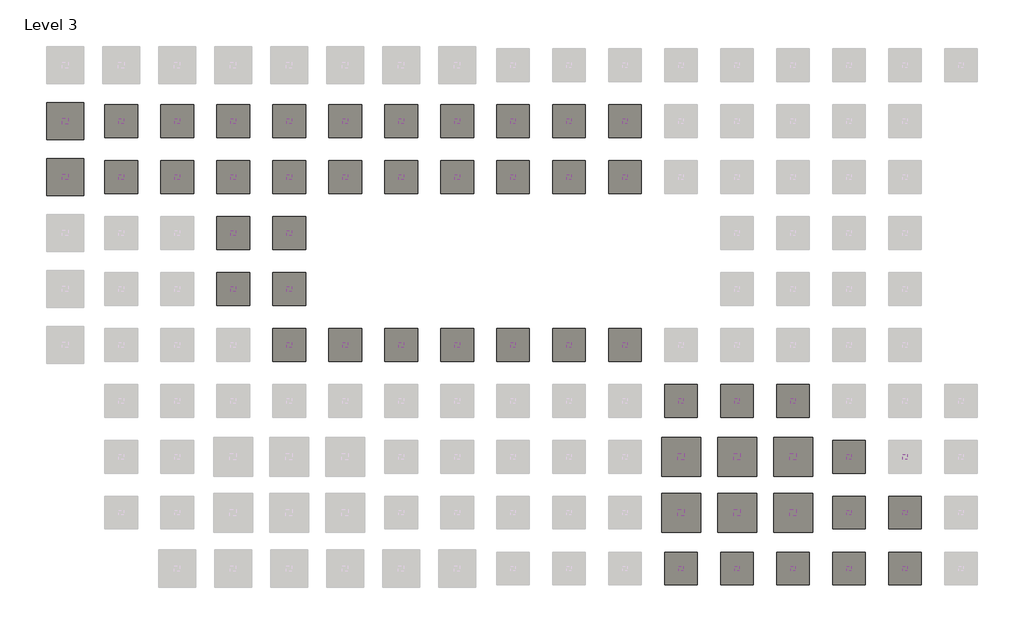
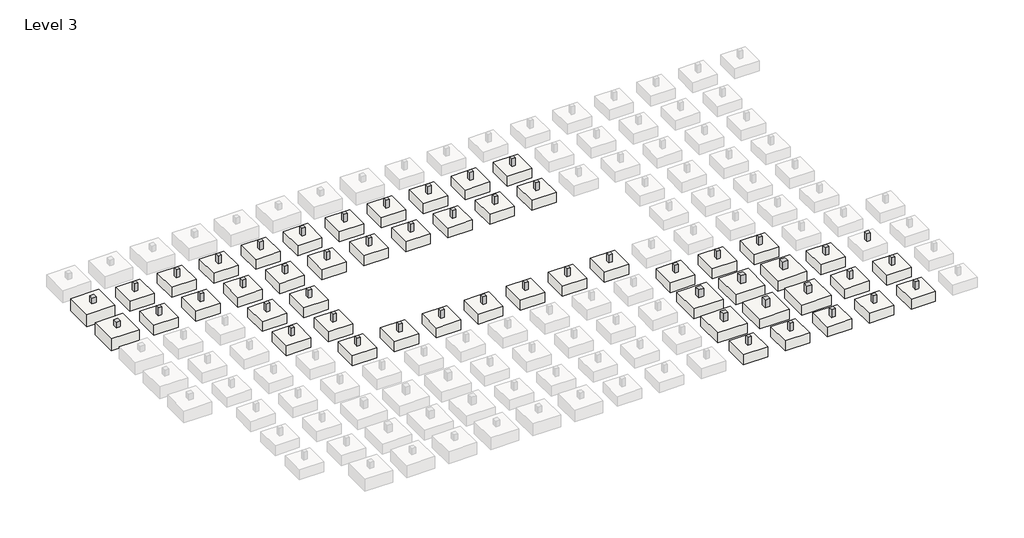
# One storey, part 2 of 3: 51 columns, 50 slabs.
"""IFC4 building model written with IfcOpenShell, lengths in millimetres."""

import ifcopenshell
import ifcopenshell.guid

model = None  # the IFC model being written
_history = None  # IfcOwnerHistory: only IFC2X3 demands one
_inside = {}  # id of a spatial element -> (the spatial element, [elements in it])
_under = {}  # id of a project, library or spatial element -> (it, [spatial elements below it])
_declared = {}  # id of a project -> (the project, [libraries it declares])
_typed = {}  # id of a type object -> (the type object, [elements of that type])
_made_of = {}  # id of a material, layer set ... -> (it, [elements and type objects made of it])


def new_model(schema):
    """Start an empty IFC model of exactly this schema.

    Asked for "IFC4X3", IfcOpenShell would pick the latest addendum, in which some entities
    have other attributes; the version numbers below select the first issue.
    IFC2X3 requires an IfcOwnerHistory on every rooted entity: one is made here for all.
    """
    global model, _history
    if schema == "IFC4X3":
        model = ifcopenshell.file(schema_version=(4, 3, 0, 0))
    else:
        model = ifcopenshell.file(schema=schema)
    _inside.clear()
    _under.clear()
    _declared.clear()
    _typed.clear()
    _made_of.clear()
    _history = None
    if model.schema == "IFC2X3":
        org = make("IfcOrganization", Name="unknown")
        user = make(
            "IfcPersonAndOrganization",
            ThePerson=make("IfcPerson", FamilyName="unknown"),
            TheOrganization=org,
        )
        app = make(
            "IfcApplication",
            ApplicationDeveloper=org,
            Version="unknown",
            ApplicationFullName="unknown",
            ApplicationIdentifier="unknown",
        )
        _history = make(
            "IfcOwnerHistory",
            OwningUser=user,
            OwningApplication=app,
            ChangeAction="ADDED",
            CreationDate=0,
        )
    return model


def make(cls, **values):
    """One entity of the class cls with the attributes given. An attribute that is None is left unset."""
    return model.create_entity(
        cls, **{name: value for name, value in values.items() if value is not None}
    )


def rooted(cls, **values):
    """An entity with a GlobalId (a new one), such as an element, a storey or a relation."""
    return make(cls, GlobalId=ifcopenshell.guid.new(), OwnerHistory=_history, **values)


def si_unit(unit_type, name, prefix=None):
    """IfcSIUnit, for example si_unit("LENGTHUNIT", "METRE", prefix="MILLI")."""
    return make("IfcSIUnit", UnitType=unit_type, Prefix=prefix, Name=name)


def assignment(units):
    """IfcUnitAssignment: the units of a project."""
    return None if units is None else make("IfcUnitAssignment", Units=units)


def point(xyz):
    """IfcCartesianPoint."""
    return None if xyz is None else make("IfcCartesianPoint", Coordinates=xyz)


def direction(xyz):
    """IfcDirection."""
    return None if xyz is None else make("IfcDirection", DirectionRatios=xyz)


def frame(location, z_axis=None, x_axis=None):
    """IfcAxis2Placement3D, a coordinate frame: its origin and axes. An axis left out is left unset."""
    return make(
        "IfcAxis2Placement3D",
        Location=point(location),
        Axis=direction(z_axis),
        RefDirection=direction(x_axis),
    )


def origin():
    """The frame at (0, 0, 0) with its axes left unset."""
    return frame((0.0, 0.0, 0.0))


def origin_with_axes():
    """The frame at (0, 0, 0) with the z axis (0, 0, 1) and the x axis (1, 0, 0) written out."""
    return frame((0.0, 0.0, 0.0), z_axis=(0.0, 0.0, 1.0), x_axis=(1.0, 0.0, 0.0))


def place(relative_to, where):
    """IfcLocalPlacement: puts the frame where relative to a parent placement (None: the world)."""
    return make(
        "IfcLocalPlacement", PlacementRelTo=relative_to, RelativePlacement=where
    )


def context(
    kind, dimensions, precision=None, world=None, true_north=None, identifier=None
):
    """IfcGeometricRepresentationContext, for example the 3D "Model" context."""
    return make(
        "IfcGeometricRepresentationContext",
        ContextIdentifier=identifier,
        ContextType=kind,
        CoordinateSpaceDimension=dimensions,
        Precision=precision,
        WorldCoordinateSystem=world,
        TrueNorth=true_north,
    )


def project(units=None, contexts=None):
    """IfcProject with its units and contexts."""
    return rooted(
        "IfcProject",
        Name="project",
        RepresentationContexts=contexts,
        UnitsInContext=assignment(units),
    )


def spatial(cls, under=None, at=None, **own):
    """A site, building, storey or space (cls), placed at a placement, below another one or the project."""
    s = rooted(cls, ObjectPlacement=at, **own)
    if under is not None:
        _under.setdefault(under.id(), (under, []))[1].append(s)
    return s


def polyline(points):
    """IfcPolyline through the points."""
    return make("IfcPolyline", Points=[point(p) for p in points])


def outline(outer, holes=None, kind="AREA"):
    """IfcArbitraryClosedProfileDef: a profile drawn as a closed curve; with holes, ...WithVoids."""
    if holes is None:
        return make("IfcArbitraryClosedProfileDef", ProfileType=kind, OuterCurve=outer)
    return make(
        "IfcArbitraryProfileDefWithVoids",
        ProfileType=kind,
        OuterCurve=outer,
        InnerCurves=holes,
    )


def extrude(swept, where, along, depth):
    """IfcExtrudedAreaSolid: the profile swept, set in the frame where, extruded along a direction by depth."""
    return make(
        "IfcExtrudedAreaSolid",
        SweptArea=swept,
        Position=where,
        ExtrudedDirection=direction(along),
        Depth=depth,
    )


def shape(context_of_items, identifier, shape_type, items):
    """IfcShapeRepresentation: the items that make up one representation, for example the "Body"."""
    return make(
        "IfcShapeRepresentation",
        ContextOfItems=context_of_items,
        RepresentationIdentifier=identifier,
        RepresentationType=shape_type,
        Items=items,
    )


def source(mapping_origin, context_of_items, identifier, shape_type, items):
    """IfcRepresentationMap: a shape defined once, which mapped items show again and again."""
    return make(
        "IfcRepresentationMap",
        MappingOrigin=mapping_origin,
        MappedRepresentation=shape(context_of_items, identifier, shape_type, items),
    )


def transform(
    local_origin,
    x_axis=None,
    y_axis=None,
    z_axis=None,
    scale=None,
    scale2=None,
    scale3=None,
    uniform=True,
):
    """IfcCartesianTransformationOperator3D, or its non-uniform kind. x_axis, y_axis, z_axis: its Axis1, 2, 3."""
    if uniform:
        return make(
            "IfcCartesianTransformationOperator3D",
            Axis1=direction(x_axis),
            Axis2=direction(y_axis),
            LocalOrigin=point(local_origin),
            Scale=scale,
            Axis3=direction(z_axis),
        )
    return make(
        "IfcCartesianTransformationOperator3DnonUniform",
        Axis1=direction(x_axis),
        Axis2=direction(y_axis),
        LocalOrigin=point(local_origin),
        Scale=scale,
        Axis3=direction(z_axis),
        Scale2=scale2,
        Scale3=scale3,
    )


def mapped(mapping_source, mapping_target):
    """IfcMappedItem: shows the shape of a source again, moved by a transform."""
    return make(
        "IfcMappedItem", MappingSource=mapping_source, MappingTarget=mapping_target
    )


def made_of(thing, what):
    """Note that an element or type object is made of a material, layer set ...; save() writes the relation."""
    if what is not None:
        _made_of.setdefault(what.id(), (what, []))[1].append(thing)
    return thing


def element(
    cls,
    number,
    at=None,
    inside=None,
    cuts=None,
    type_object=None,
    material=None,
    context=None,
    identifier="Body",
    shape_type=None,
    held_by="IfcProductDefinitionShape",
    body=None,
    shapes=None,
    **own,
):
    """One element of the class cls, such as IfcWall. Its Tag is "e" and its number.

    at: its placement. inside: the storey or other place that contains it. cuts: it is an
    opening in that element (IfcRelVoidsElement). A single representation is given by context,
    identifier, shape_type and body (its items); several are given by shapes. held_by: the class
    of the entity that holds the representations. save() writes the other relations.
    """
    e = rooted(cls, Tag="e%d" % number, ObjectPlacement=at, **own)
    if body is not None:
        shapes = [shape(context, identifier, shape_type, body)]
    if shapes is not None:
        e.Representation = make(held_by, Representations=shapes)
    if inside is not None:
        _inside.setdefault(inside.id(), (inside, []))[1].append(e)
    if cuts is not None:
        rooted(
            "IfcRelVoidsElement", RelatingBuildingElement=cuts, RelatedOpeningElement=e
        )
    if type_object is not None:
        _typed.setdefault(type_object.id(), (type_object, []))[1].append(e)
    return made_of(e, material)


def aggregate(whole, parts):
    """IfcRelAggregates: a whole, such as a stair, and the parts it consists of."""
    return rooted("IfcRelAggregates", RelatingObject=whole, RelatedObjects=parts)


def save(model, path):
    """Write the relations noted so far, then the file.

    IfcRelAggregates (storeys below a building ...), IfcRelContainedInSpatialStructure (elements
    in a storey), IfcRelDefinesByType, IfcRelAssociatesMaterial and IfcRelDeclares: one each for
    every whole, place, type object, material and project.
    """
    for whole, parts in _under.values():
        aggregate(whole, parts)
    for where, things in _inside.values():
        rooted(
            "IfcRelContainedInSpatialStructure",
            RelatedElements=things,
            RelatingStructure=where,
        )
    for kind, things in _typed.values():
        rooted("IfcRelDefinesByType", RelatedObjects=things, RelatingType=kind)
    for what, things in _made_of.values():
        rooted("IfcRelAssociatesMaterial", RelatedObjects=things, RelatingMaterial=what)
    for by, libraries in _declared.values():
        rooted("IfcRelDeclares", RelatingContext=by, RelatedDefinitions=libraries)
    model.write(path)


def cl111_concrete_rectangular_column_cl111_500x500_13a722a7(model_context):
    return source(origin(), model_context, "Body", "SweptSolid", [
        extrude(outline(polyline([(250.0, 250.0), (250.0, -250.0), (-250.0, -250.0), (-250.0, 250.0), (250.0, 250.0)])), frame((0.0, 0.0, -1200.0), z_axis=(0.0, 0.0, 1.0), x_axis=(1.0, 0.0, 0.0)), (0.0, 0.0, 1.0), 1200.0),
    ])


def cl111_concrete_rectangular_column_cl111_700x700_c1bab047(model_context):
    return source(origin(), model_context, "Body", "SweptSolid", [
        extrude(outline(polyline([(350.0, 350.0), (350.0, -350.0), (-350.0, -350.0), (-350.0, 350.0), (350.0, 350.0)])), frame((0.0, 0.0, -1200.0), z_axis=(0.0, 0.0, 1.0), x_axis=(1.0, 0.0, 0.0)), (0.0, 0.0, 1.0), 1200.0),
    ])


def ft111_footing_rectangular_ft111_3500x3500_d0491e67(model_context):
    return source(origin(), model_context, "Body", "SweptSolid", [
        extrude(outline(polyline([(1750.0, 1750.0), (1750.0, -1750.0), (-1750.0, -1750.0), (-1750.0, 1750.0), (1750.0, 1750.0)])), origin_with_axes(), (0.0, 0.0, 1.0), 1500.0),
    ])


def ft111_footing_rectangular_ft111_4200x4200_1dfe1a53(model_context):
    return source(origin(), model_context, "Body", "SweptSolid", [
        extrude(outline(polyline([(2100.0, 2100.0), (2100.0, -2100.0), (-2100.0, -2100.0), (-2100.0, 2100.0), (2100.0, 2100.0)])), origin_with_axes(), (0.0, 0.0, 1.0), 1500.0),
    ])


model = new_model("IFC4")

# Units and contexts
model_context = context("Model", 3, world=origin())
ifc_project = project(units=[si_unit("LENGTHUNIT", "METRE", prefix="MILLI")], contexts=[model_context])

# Site, building, storey
site = spatial("IfcSite", under=ifc_project)
building = spatial("IfcBuilding", under=site)
storey = spatial("IfcBuildingStorey", under=building, Name="Level 3", Elevation=-2700.0)

# Columns
placement = place(None, origin())
element("IfcColumn", 1, ObjectType="CL111_Concrete-Rectangular-Column : CL111_500x500", at=placement, inside=storey, context=model_context, shape_type="SweptSolid", body=[
    extrude(outline(polyline([(84250.0, -53750.0), (84250.0, -54250.0), (83750.0, -54250.0), (83750.0, -53750.0), (84250.0, -53750.0)])), frame((0.0, 0.0, -1200.0), z_axis=(0.0, 0.0, 1.0), x_axis=(1.0, 0.0, 0.0)), (0.0, 0.0, 1.0), 1200.0),
])
element("IfcColumn", 2, ObjectType="CL111_Concrete-Rectangular-Column : CL111_500x500", at=placement, inside=storey, context=model_context, shape_type="SweptSolid", body=[
    extrude(outline(polyline([(90250.0, -53750.0), (90250.0, -54250.0), (89750.0, -54250.0), (89750.0, -53750.0), (90250.0, -53750.0)])), frame((0.0, 0.0, -1200.0), z_axis=(0.0, 0.0, 1.0), x_axis=(1.0, 0.0, 0.0)), (0.0, 0.0, 1.0), 1200.0),
])
element("IfcColumn", 3, ObjectType="CL111_Concrete-Rectangular-Column : CL111_500x500", at=placement, inside=storey, context=model_context, shape_type="SweptSolid", body=[
    extrude(outline(polyline([(72250.0, -53750.0), (72250.0, -54250.0), (71750.0, -54250.0), (71750.0, -53750.0), (72250.0, -53750.0)])), frame((0.0, 0.0, -1200.0), z_axis=(0.0, 0.0, 1.0), x_axis=(1.0, 0.0, 0.0)), (0.0, 0.0, 1.0), 1200.0),
])
element("IfcColumn", 4, ObjectType="CL111_Concrete-Rectangular-Column : CL111_500x500", at=placement, inside=storey, context=model_context, shape_type="SweptSolid", body=[
    extrude(outline(polyline([(78250.0, -53750.0), (78250.0, -54250.0), (77750.0, -54250.0), (77750.0, -53750.0), (78250.0, -53750.0)])), frame((0.0, 0.0, -1200.0), z_axis=(0.0, 0.0, 1.0), x_axis=(1.0, 0.0, 0.0)), (0.0, 0.0, 1.0), 1200.0),
])
element("IfcColumn", 5, ObjectType="CL111_Concrete-Rectangular-Column : CL111_500x500", at=placement, inside=storey, context=model_context, shape_type="SweptSolid", body=[
    extrude(outline(polyline([(66250.0, -53750.0), (66250.0, -54250.0), (65750.0, -54250.0), (65750.0, -53750.0), (66250.0, -53750.0)])), frame((0.0, 0.0, -1200.0), z_axis=(0.0, 0.0, 1.0), x_axis=(1.0, 0.0, 0.0)), (0.0, 0.0, 1.0), 1200.0),
])
cl111_concrete_rectangular_column_cl111_500x500_shape = cl111_concrete_rectangular_column_cl111_500x500_13a722a7(model_context)
element("IfcColumn", 6, ObjectType="CL111_Concrete-Rectangular-Column : CL111_500x500", at=placement, inside=storey, context=model_context, shape_type="MappedRepresentation", body=[
    mapped(cl111_concrete_rectangular_column_cl111_500x500_shape, transform((54000.0, -30000.0, 0.0), x_axis=(1.0, 0.0, 0.0), y_axis=(0.0, 1.0, 0.0), z_axis=(0.0, 0.0, 1.0))),
])
element("IfcColumn", 7, ObjectType="CL111_Concrete-Rectangular-Column : CL111_500x500", at=placement, inside=storey, context=model_context, shape_type="MappedRepresentation", body=[
    mapped(cl111_concrete_rectangular_column_cl111_500x500_shape, transform((54000.0, -12000.0, 0.0), x_axis=(1.0, 0.0, 0.0), y_axis=(0.0, 1.0, 0.0), z_axis=(0.0, 0.0, 1.0))),
])
element("IfcColumn", 8, ObjectType="CL111_Concrete-Rectangular-Column : CL111_500x500", at=placement, inside=storey, context=model_context, shape_type="MappedRepresentation", body=[
    mapped(cl111_concrete_rectangular_column_cl111_500x500_shape, transform((54000.0, -6000.0, 0.0), x_axis=(1.0, 0.0, 0.0), y_axis=(0.0, 1.0, 0.0), z_axis=(0.0, 0.0, 1.0))),
])
element("IfcColumn", 9, ObjectType="CL111_Concrete-Rectangular-Column : CL111_500x500", at=placement, inside=storey, context=model_context, shape_type="MappedRepresentation", body=[
    mapped(cl111_concrete_rectangular_column_cl111_500x500_shape, transform((84000.0, -48000.0, 0.0), x_axis=(1.0, 0.0, 0.0), y_axis=(0.0, 1.0, 0.0), z_axis=(0.0, 0.0, 1.0))),
])
element("IfcColumn", 10, ObjectType="CL111_Concrete-Rectangular-Column : CL111_500x500", at=placement, inside=storey, context=model_context, shape_type="MappedRepresentation", body=[
    mapped(cl111_concrete_rectangular_column_cl111_500x500_shape, transform((84000.0, -42000.0, 0.0), x_axis=(1.0, 0.0, 0.0), y_axis=(0.0, 1.0, 0.0), z_axis=(0.0, 0.0, 1.0))),
])
element("IfcColumn", 11, ObjectType="CL111_Concrete-Rectangular-Column : CL111_500x500", at=placement, inside=storey, context=model_context, shape_type="MappedRepresentation", body=[
    mapped(cl111_concrete_rectangular_column_cl111_500x500_shape, transform((18000.0, -24000.0, 0.0), x_axis=(1.0, 0.0, 0.0), y_axis=(0.0, 1.0, 0.0), z_axis=(0.0, 0.0, 1.0))),
])
element("IfcColumn", 12, ObjectType="CL111_Concrete-Rectangular-Column : CL111_500x500", at=placement, inside=storey, context=model_context, shape_type="MappedRepresentation", body=[
    mapped(cl111_concrete_rectangular_column_cl111_500x500_shape, transform((24000.0, -24000.0, 0.0), x_axis=(1.0, 0.0, 0.0), y_axis=(0.0, 1.0, 0.0), z_axis=(0.0, 0.0, 1.0))),
])
element("IfcColumn", 13, ObjectType="CL111_Concrete-Rectangular-Column : CL111_500x500", at=placement, inside=storey, context=model_context, shape_type="MappedRepresentation", body=[
    mapped(cl111_concrete_rectangular_column_cl111_500x500_shape, transform((24000.0, -18000.0, 0.0), x_axis=(1.0, 0.0, 0.0), y_axis=(0.0, 1.0, 0.0), z_axis=(0.0, 0.0, 1.0))),
])
element("IfcColumn", 14, ObjectType="CL111_Concrete-Rectangular-Column : CL111_500x500", at=placement, inside=storey, context=model_context, shape_type="MappedRepresentation", body=[
    mapped(cl111_concrete_rectangular_column_cl111_500x500_shape, transform((18000.0, -18000.0, 0.0), x_axis=(1.0, 0.0, 0.0), y_axis=(0.0, 1.0, 0.0), z_axis=(0.0, 0.0, 1.0))),
])
element("IfcColumn", 15, ObjectType="CL111_Concrete-Rectangular-Column : CL111_500x500", at=placement, inside=storey, context=model_context, shape_type="MappedRepresentation", body=[
    mapped(cl111_concrete_rectangular_column_cl111_500x500_shape, transform((36000.0, -30000.0, 0.0), x_axis=(1.0, 0.0, 0.0), y_axis=(0.0, 1.0, 0.0), z_axis=(0.0, 0.0, 1.0))),
])
element("IfcColumn", 16, ObjectType="CL111_Concrete-Rectangular-Column : CL111_500x500", at=placement, inside=storey, context=model_context, shape_type="MappedRepresentation", body=[
    mapped(cl111_concrete_rectangular_column_cl111_500x500_shape, transform((30000.0, -30000.0, 0.0), x_axis=(1.0, 0.0, 0.0), y_axis=(0.0, 1.0, 0.0), z_axis=(0.0, 0.0, 1.0))),
])
element("IfcColumn", 17, ObjectType="CL111_Concrete-Rectangular-Column : CL111_500x500", at=placement, inside=storey, context=model_context, shape_type="MappedRepresentation", body=[
    mapped(cl111_concrete_rectangular_column_cl111_500x500_shape, transform((24000.0, -30000.0, 0.0), x_axis=(1.0, 0.0, 0.0), y_axis=(0.0, 1.0, 0.0), z_axis=(0.0, 0.0, 1.0))),
])
element("IfcColumn", 18, ObjectType="CL111_Concrete-Rectangular-Column : CL111_500x500", at=placement, inside=storey, context=model_context, shape_type="MappedRepresentation", body=[
    mapped(cl111_concrete_rectangular_column_cl111_500x500_shape, transform((48000.0, -30000.0, 0.0), x_axis=(1.0, 0.0, 0.0), y_axis=(0.0, 1.0, 0.0), z_axis=(0.0, 0.0, 1.0))),
])
element("IfcColumn", 19, ObjectType="CL111_Concrete-Rectangular-Column : CL111_500x500", at=placement, inside=storey, context=model_context, shape_type="MappedRepresentation", body=[
    mapped(cl111_concrete_rectangular_column_cl111_500x500_shape, transform((42000.0, -30000.0, 0.0), x_axis=(1.0, 0.0, 0.0), y_axis=(0.0, 1.0, 0.0), z_axis=(0.0, 0.0, 1.0))),
])
element("IfcColumn", 20, ObjectType="CL111_Concrete-Rectangular-Column : CL111_500x500", at=placement, inside=storey, context=model_context, shape_type="MappedRepresentation", body=[
    mapped(cl111_concrete_rectangular_column_cl111_500x500_shape, transform((30000.0, -12000.0, 0.0), x_axis=(1.0, 0.0, 0.0), y_axis=(0.0, 1.0, 0.0), z_axis=(0.0, 0.0, 1.0))),
])
element("IfcColumn", 21, ObjectType="CL111_Concrete-Rectangular-Column : CL111_500x500", at=placement, inside=storey, context=model_context, shape_type="MappedRepresentation", body=[
    mapped(cl111_concrete_rectangular_column_cl111_500x500_shape, transform((36000.0, -12000.0, 0.0), x_axis=(1.0, 0.0, 0.0), y_axis=(0.0, 1.0, 0.0), z_axis=(0.0, 0.0, 1.0))),
])
element("IfcColumn", 22, ObjectType="CL111_Concrete-Rectangular-Column : CL111_500x500", at=placement, inside=storey, context=model_context, shape_type="MappedRepresentation", body=[
    mapped(cl111_concrete_rectangular_column_cl111_500x500_shape, transform((18000.0, -12000.0, 0.0), x_axis=(1.0, 0.0, 0.0), y_axis=(0.0, 1.0, 0.0), z_axis=(0.0, 0.0, 1.0))),
])
element("IfcColumn", 23, ObjectType="CL111_Concrete-Rectangular-Column : CL111_500x500", at=placement, inside=storey, context=model_context, shape_type="MappedRepresentation", body=[
    mapped(cl111_concrete_rectangular_column_cl111_500x500_shape, transform((24000.0, -12000.0, 0.0), x_axis=(1.0, 0.0, 0.0), y_axis=(0.0, 1.0, 0.0), z_axis=(0.0, 0.0, 1.0))),
])
element("IfcColumn", 24, ObjectType="CL111_Concrete-Rectangular-Column : CL111_500x500", at=placement, inside=storey, context=model_context, shape_type="MappedRepresentation", body=[
    mapped(cl111_concrete_rectangular_column_cl111_500x500_shape, transform((6000.0, -12000.0, 0.0), x_axis=(1.0, 0.0, 0.0), y_axis=(0.0, 1.0, 0.0), z_axis=(0.0, 0.0, 1.0))),
])
element("IfcColumn", 25, ObjectType="CL111_Concrete-Rectangular-Column : CL111_500x500", at=placement, inside=storey, context=model_context, shape_type="MappedRepresentation", body=[
    mapped(cl111_concrete_rectangular_column_cl111_500x500_shape, transform((12000.0, -12000.0, 0.0), x_axis=(1.0, 0.0, 0.0), y_axis=(0.0, 1.0, 0.0), z_axis=(0.0, 0.0, 1.0))),
])
element("IfcColumn", 26, ObjectType="CL111_Concrete-Rectangular-Column : CL111_500x500", at=placement, inside=storey, context=model_context, shape_type="MappedRepresentation", body=[
    mapped(cl111_concrete_rectangular_column_cl111_500x500_shape, transform((42000.0, -12000.0, 0.0), x_axis=(1.0, 0.0, 0.0), y_axis=(0.0, 1.0, 0.0), z_axis=(0.0, 0.0, 1.0))),
])
element("IfcColumn", 27, ObjectType="CL111_Concrete-Rectangular-Column : CL111_500x500", at=placement, inside=storey, context=model_context, shape_type="MappedRepresentation", body=[
    mapped(cl111_concrete_rectangular_column_cl111_500x500_shape, transform((48000.0, -12000.0, 0.0), x_axis=(1.0, 0.0, 0.0), y_axis=(0.0, 1.0, 0.0), z_axis=(0.0, 0.0, 1.0))),
])
element("IfcColumn", 28, ObjectType="CL111_Concrete-Rectangular-Column : CL111_500x500", at=placement, inside=storey, context=model_context, shape_type="MappedRepresentation", body=[
    mapped(cl111_concrete_rectangular_column_cl111_500x500_shape, transform((36000.0, -6000.0, 0.0), x_axis=(1.0, 0.0, 0.0), y_axis=(0.0, 1.0, 0.0), z_axis=(0.0, 0.0, 1.0))),
])
element("IfcColumn", 29, ObjectType="CL111_Concrete-Rectangular-Column : CL111_500x500", at=placement, inside=storey, context=model_context, shape_type="MappedRepresentation", body=[
    mapped(cl111_concrete_rectangular_column_cl111_500x500_shape, transform((30000.0, -6000.0, 0.0), x_axis=(1.0, 0.0, 0.0), y_axis=(0.0, 1.0, 0.0), z_axis=(0.0, 0.0, 1.0))),
])
element("IfcColumn", 30, ObjectType="CL111_Concrete-Rectangular-Column : CL111_500x500", at=placement, inside=storey, context=model_context, shape_type="MappedRepresentation", body=[
    mapped(cl111_concrete_rectangular_column_cl111_500x500_shape, transform((24000.0, -6000.0, 0.0), x_axis=(1.0, 0.0, 0.0), y_axis=(0.0, 1.0, 0.0), z_axis=(0.0, 0.0, 1.0))),
])
element("IfcColumn", 31, ObjectType="CL111_Concrete-Rectangular-Column : CL111_500x500", at=placement, inside=storey, context=model_context, shape_type="MappedRepresentation", body=[
    mapped(cl111_concrete_rectangular_column_cl111_500x500_shape, transform((18000.0, -6000.0, 0.0), x_axis=(1.0, 0.0, 0.0), y_axis=(0.0, 1.0, 0.0), z_axis=(0.0, 0.0, 1.0))),
])
element("IfcColumn", 32, ObjectType="CL111_Concrete-Rectangular-Column : CL111_500x500", at=placement, inside=storey, context=model_context, shape_type="MappedRepresentation", body=[
    mapped(cl111_concrete_rectangular_column_cl111_500x500_shape, transform((12000.0, -6000.0, 0.0), x_axis=(1.0, 0.0, 0.0), y_axis=(0.0, 1.0, 0.0), z_axis=(0.0, 0.0, 1.0))),
])
element("IfcColumn", 33, ObjectType="CL111_Concrete-Rectangular-Column : CL111_500x500", at=placement, inside=storey, context=model_context, shape_type="MappedRepresentation", body=[
    mapped(cl111_concrete_rectangular_column_cl111_500x500_shape, transform((6000.0, -6000.0, 0.0), x_axis=(1.0, 0.0, 0.0), y_axis=(0.0, 1.0, 0.0), z_axis=(0.0, 0.0, 1.0))),
])
element("IfcColumn", 34, ObjectType="CL111_Concrete-Rectangular-Column : CL111_500x500", at=placement, inside=storey, context=model_context, shape_type="MappedRepresentation", body=[
    mapped(cl111_concrete_rectangular_column_cl111_500x500_shape, transform((48000.0, -6000.0, 0.0), x_axis=(1.0, 0.0, 0.0), y_axis=(0.0, 1.0, 0.0), z_axis=(0.0, 0.0, 1.0))),
])
element("IfcColumn", 35, ObjectType="CL111_Concrete-Rectangular-Column : CL111_500x500", at=placement, inside=storey, context=model_context, shape_type="MappedRepresentation", body=[
    mapped(cl111_concrete_rectangular_column_cl111_500x500_shape, transform((42000.0, -6000.0, 0.0), x_axis=(1.0, 0.0, 0.0), y_axis=(0.0, 1.0, 0.0), z_axis=(0.0, 0.0, 1.0))),
])
element("IfcColumn", 36, ObjectType="CL111_Concrete-Rectangular-Column : CL111_500x500", at=placement, inside=storey, context=model_context, shape_type="MappedRepresentation", body=[
    mapped(cl111_concrete_rectangular_column_cl111_500x500_shape, transform((90000.0, -48000.0, 0.0), x_axis=(1.0, 0.0, 0.0), y_axis=(0.0, 1.0, 0.0), z_axis=(0.0, 0.0, 1.0))),
])
element("IfcColumn", 37, ObjectType="CL111_Concrete-Rectangular-Column : CL111_500x500", at=placement, inside=storey, context=model_context, shape_type="MappedRepresentation", body=[
    mapped(cl111_concrete_rectangular_column_cl111_500x500_shape, transform((90000.0, -42000.0, 0.0), x_axis=(1.0, 0.0, 0.0), y_axis=(0.0, 1.0, 0.0), z_axis=(0.0, 0.0, 1.0))),
])
element("IfcColumn", 38, ObjectType="CL111_Concrete-Rectangular-Column : CL111_500x500", at=placement, inside=storey, context=model_context, shape_type="MappedRepresentation", body=[
    mapped(cl111_concrete_rectangular_column_cl111_500x500_shape, transform((72000.0, -36000.0, 0.0), x_axis=(1.0, 0.0, 0.0), y_axis=(0.0, 1.0, 0.0), z_axis=(0.0, 0.0, 1.0))),
])
element("IfcColumn", 39, ObjectType="CL111_Concrete-Rectangular-Column : CL111_500x500", at=placement, inside=storey, context=model_context, shape_type="MappedRepresentation", body=[
    mapped(cl111_concrete_rectangular_column_cl111_500x500_shape, transform((78000.0, -36000.0, 0.0), x_axis=(1.0, 0.0, 0.0), y_axis=(0.0, 1.0, 0.0), z_axis=(0.0, 0.0, 1.0))),
])
element("IfcColumn", 40, ObjectType="CL111_Concrete-Rectangular-Column : CL111_500x500", at=placement, inside=storey, context=model_context, shape_type="MappedRepresentation", body=[
    mapped(cl111_concrete_rectangular_column_cl111_500x500_shape, transform((60000.0, -30000.0, 0.0), x_axis=(1.0, 0.0, 0.0), y_axis=(0.0, 1.0, 0.0), z_axis=(0.0, 0.0, 1.0))),
])
element("IfcColumn", 41, ObjectType="CL111_Concrete-Rectangular-Column : CL111_500x500", at=placement, inside=storey, context=model_context, shape_type="MappedRepresentation", body=[
    mapped(cl111_concrete_rectangular_column_cl111_500x500_shape, transform((60000.0, -12000.0, 0.0), x_axis=(1.0, 0.0, 0.0), y_axis=(0.0, 1.0, 0.0), z_axis=(0.0, 0.0, 1.0))),
])
element("IfcColumn", 42, ObjectType="CL111_Concrete-Rectangular-Column : CL111_500x500", at=placement, inside=storey, context=model_context, shape_type="MappedRepresentation", body=[
    mapped(cl111_concrete_rectangular_column_cl111_500x500_shape, transform((60000.0, -6000.0, 0.0), x_axis=(1.0, 0.0, 0.0), y_axis=(0.0, 1.0, 0.0), z_axis=(0.0, 0.0, 1.0))),
])
element("IfcColumn", 43, ObjectType="CL111_Concrete-Rectangular-Column : CL111_500x500", at=placement, inside=storey, context=model_context, shape_type="MappedRepresentation", body=[
    mapped(cl111_concrete_rectangular_column_cl111_500x500_shape, transform((66000.0, -36000.0, 0.0), x_axis=(1.0, 0.0, 0.0), y_axis=(0.0, 1.0, 0.0), z_axis=(0.0, 0.0, 1.0))),
])
element("IfcColumn", 44, ObjectType="CL111_Concrete-Rectangular-Column : CL111_600x600", at=placement, inside=storey, context=model_context, shape_type="SweptSolid", body=[
    extrude(outline(polyline([(300.0, -11700.0), (300.0, -12300.0), (-300.0, -12300.0), (-300.0, -11700.0), (300.0, -11700.0)])), frame((0.0, 0.0, -900.0), z_axis=(0.0, 0.0, 1.0), x_axis=(1.0, 0.0, 0.0)), (0.0, 0.0, 1.0), 900.0),
])
element("IfcColumn", 45, ObjectType="CL111_Concrete-Rectangular-Column : CL111_600x600", at=placement, inside=storey, context=model_context, shape_type="SweptSolid", body=[
    extrude(outline(polyline([(300.0, -5700.0), (300.0, -6300.0), (-300.0, -6300.0), (-300.0, -5700.0), (300.0, -5700.0)])), frame((0.0, 0.0, -900.0), z_axis=(0.0, 0.0, 1.0), x_axis=(1.0, 0.0, 0.0)), (0.0, 0.0, 1.0), 900.0),
])
cl111_concrete_rectangular_column_cl111_700x700_shape = cl111_concrete_rectangular_column_cl111_700x700_c1bab047(model_context)
element("IfcColumn", 46, ObjectType="CL111_Concrete-Rectangular-Column : CL111_700x700", at=placement, inside=storey, context=model_context, shape_type="MappedRepresentation", body=[
    mapped(cl111_concrete_rectangular_column_cl111_700x700_shape, transform((72000.0, -48000.0, 0.0), x_axis=(1.0, 0.0, 0.0), y_axis=(0.0, 1.0, 0.0), z_axis=(0.0, 0.0, 1.0))),
])
element("IfcColumn", 47, ObjectType="CL111_Concrete-Rectangular-Column : CL111_700x700", at=placement, inside=storey, context=model_context, shape_type="MappedRepresentation", body=[
    mapped(cl111_concrete_rectangular_column_cl111_700x700_shape, transform((72000.0, -42000.0, 0.0), x_axis=(1.0, 0.0, 0.0), y_axis=(0.0, 1.0, 0.0), z_axis=(0.0, 0.0, 1.0))),
])
element("IfcColumn", 48, ObjectType="CL111_Concrete-Rectangular-Column : CL111_700x700", at=placement, inside=storey, context=model_context, shape_type="MappedRepresentation", body=[
    mapped(cl111_concrete_rectangular_column_cl111_700x700_shape, transform((78000.0, -48000.0, 0.0), x_axis=(1.0, 0.0, 0.0), y_axis=(0.0, 1.0, 0.0), z_axis=(0.0, 0.0, 1.0))),
])
element("IfcColumn", 49, ObjectType="CL111_Concrete-Rectangular-Column : CL111_700x700", at=placement, inside=storey, context=model_context, shape_type="MappedRepresentation", body=[
    mapped(cl111_concrete_rectangular_column_cl111_700x700_shape, transform((78000.0, -42000.0, 0.0), x_axis=(1.0, 0.0, 0.0), y_axis=(0.0, 1.0, 0.0), z_axis=(0.0, 0.0, 1.0))),
])
element("IfcColumn", 50, ObjectType="CL111_Concrete-Rectangular-Column : CL111_700x700", at=placement, inside=storey, context=model_context, shape_type="MappedRepresentation", body=[
    mapped(cl111_concrete_rectangular_column_cl111_700x700_shape, transform((66000.0, -48000.0, 0.0), x_axis=(1.0, 0.0, 0.0), y_axis=(0.0, 1.0, 0.0), z_axis=(0.0, 0.0, 1.0))),
])
element("IfcColumn", 51, ObjectType="CL111_Concrete-Rectangular-Column : CL111_700x700", at=placement, inside=storey, context=model_context, shape_type="MappedRepresentation", body=[
    mapped(cl111_concrete_rectangular_column_cl111_700x700_shape, transform((66000.0, -42000.0, 0.0), x_axis=(1.0, 0.0, 0.0), y_axis=(0.0, 1.0, 0.0), z_axis=(0.0, 0.0, 1.0))),
])

# Slabs
element("IfcSlab", 52, ObjectType="FT111_Footing-Rectangular : FT111_3500x3500", at=placement, inside=storey, context=model_context, shape_type="SweptSolid", body=[
    extrude(outline(polyline([(85750.0, -52250.0), (85750.0, -55750.0), (82250.0, -55750.0), (82250.0, -52250.0), (85750.0, -52250.0)])), frame((0.0, 0.0, -2700.0), z_axis=(0.0, 0.0, 1.0), x_axis=(1.0, 0.0, 0.0)), (0.0, 0.0, 1.0), 1500.0),
])
element("IfcSlab", 53, ObjectType="FT111_Footing-Rectangular : FT111_3500x3500", at=placement, inside=storey, context=model_context, shape_type="SweptSolid", body=[
    extrude(outline(polyline([(91750.0, -52250.0), (91750.0, -55750.0), (88250.0, -55750.0), (88250.0, -52250.0), (91750.0, -52250.0)])), frame((0.0, 0.0, -2700.0), z_axis=(0.0, 0.0, 1.0), x_axis=(1.0, 0.0, 0.0)), (0.0, 0.0, 1.0), 1500.0),
])
element("IfcSlab", 54, ObjectType="FT111_Footing-Rectangular : FT111_3500x3500", at=placement, inside=storey, context=model_context, shape_type="SweptSolid", body=[
    extrude(outline(polyline([(73750.0, -52250.0), (73750.0, -55750.0), (70250.0, -55750.0), (70250.0, -52250.0), (73750.0, -52250.0)])), frame((0.0, 0.0, -2700.0), z_axis=(0.0, 0.0, 1.0), x_axis=(1.0, 0.0, 0.0)), (0.0, 0.0, 1.0), 1500.0),
])
element("IfcSlab", 55, ObjectType="FT111_Footing-Rectangular : FT111_3500x3500", at=placement, inside=storey, context=model_context, shape_type="SweptSolid", body=[
    extrude(outline(polyline([(79750.0, -52250.0), (79750.0, -55750.0), (76250.0, -55750.0), (76250.0, -52250.0), (79750.0, -52250.0)])), frame((0.0, 0.0, -2700.0), z_axis=(0.0, 0.0, 1.0), x_axis=(1.0, 0.0, 0.0)), (0.0, 0.0, 1.0), 1500.0),
])
element("IfcSlab", 56, ObjectType="FT111_Footing-Rectangular : FT111_3500x3500", at=placement, inside=storey, context=model_context, shape_type="SweptSolid", body=[
    extrude(outline(polyline([(67750.0, -52250.0), (67750.0, -55750.0), (64250.0, -55750.0), (64250.0, -52250.0), (67750.0, -52250.0)])), frame((0.0, 0.0, -2700.0), z_axis=(0.0, 0.0, 1.0), x_axis=(1.0, 0.0, 0.0)), (0.0, 0.0, 1.0), 1500.0),
])
ft111_footing_rectangular_ft111_3500x3500_shape = ft111_footing_rectangular_ft111_3500x3500_d0491e67(model_context)
element("IfcSlab", 57, ObjectType="FT111_Footing-Rectangular : FT111_3500x3500", at=placement, inside=storey, context=model_context, shape_type="MappedRepresentation", body=[
    mapped(ft111_footing_rectangular_ft111_3500x3500_shape, transform((54000.0, -30000.0, -2700.0), x_axis=(1.0, 0.0, 0.0), y_axis=(0.0, 1.0, 0.0), z_axis=(0.0, 0.0, 1.0))),
])
element("IfcSlab", 58, ObjectType="FT111_Footing-Rectangular : FT111_3500x3500", at=placement, inside=storey, context=model_context, shape_type="MappedRepresentation", body=[
    mapped(ft111_footing_rectangular_ft111_3500x3500_shape, transform((54000.0, -12000.0, -2700.0), x_axis=(1.0, 0.0, 0.0), y_axis=(0.0, 1.0, 0.0), z_axis=(0.0, 0.0, 1.0))),
])
element("IfcSlab", 59, ObjectType="FT111_Footing-Rectangular : FT111_3500x3500", at=placement, inside=storey, context=model_context, shape_type="MappedRepresentation", body=[
    mapped(ft111_footing_rectangular_ft111_3500x3500_shape, transform((54000.0, -6000.0, -2700.0), x_axis=(1.0, 0.0, 0.0), y_axis=(0.0, 1.0, 0.0), z_axis=(0.0, 0.0, 1.0))),
])
element("IfcSlab", 60, ObjectType="FT111_Footing-Rectangular : FT111_3500x3500", at=placement, inside=storey, context=model_context, shape_type="MappedRepresentation", body=[
    mapped(ft111_footing_rectangular_ft111_3500x3500_shape, transform((84000.0, -48000.0, -2700.0), x_axis=(1.0, 0.0, 0.0), y_axis=(0.0, 1.0, 0.0), z_axis=(0.0, 0.0, 1.0))),
])
element("IfcSlab", 61, ObjectType="FT111_Footing-Rectangular : FT111_3500x3500", at=placement, inside=storey, context=model_context, shape_type="MappedRepresentation", body=[
    mapped(ft111_footing_rectangular_ft111_3500x3500_shape, transform((84000.0, -42000.0, -2700.0), x_axis=(1.0, 0.0, 0.0), y_axis=(0.0, 1.0, 0.0), z_axis=(0.0, 0.0, 1.0))),
])
element("IfcSlab", 62, ObjectType="FT111_Footing-Rectangular : FT111_3500x3500", at=placement, inside=storey, context=model_context, shape_type="MappedRepresentation", body=[
    mapped(ft111_footing_rectangular_ft111_3500x3500_shape, transform((18000.0, -24000.0, -2700.0), x_axis=(1.0, 0.0, 0.0), y_axis=(0.0, 1.0, 0.0), z_axis=(0.0, 0.0, 1.0))),
])
element("IfcSlab", 63, ObjectType="FT111_Footing-Rectangular : FT111_3500x3500", at=placement, inside=storey, context=model_context, shape_type="MappedRepresentation", body=[
    mapped(ft111_footing_rectangular_ft111_3500x3500_shape, transform((24000.0, -24000.0, -2700.0), x_axis=(1.0, 0.0, 0.0), y_axis=(0.0, 1.0, 0.0), z_axis=(0.0, 0.0, 1.0))),
])
element("IfcSlab", 64, ObjectType="FT111_Footing-Rectangular : FT111_3500x3500", at=placement, inside=storey, context=model_context, shape_type="MappedRepresentation", body=[
    mapped(ft111_footing_rectangular_ft111_3500x3500_shape, transform((24000.0, -18000.0, -2700.0), x_axis=(1.0, 0.0, 0.0), y_axis=(0.0, 1.0, 0.0), z_axis=(0.0, 0.0, 1.0))),
])
element("IfcSlab", 65, ObjectType="FT111_Footing-Rectangular : FT111_3500x3500", at=placement, inside=storey, context=model_context, shape_type="MappedRepresentation", body=[
    mapped(ft111_footing_rectangular_ft111_3500x3500_shape, transform((18000.0, -18000.0, -2700.0), x_axis=(1.0, 0.0, 0.0), y_axis=(0.0, 1.0, 0.0), z_axis=(0.0, 0.0, 1.0))),
])
element("IfcSlab", 66, ObjectType="FT111_Footing-Rectangular : FT111_3500x3500", at=placement, inside=storey, context=model_context, shape_type="MappedRepresentation", body=[
    mapped(ft111_footing_rectangular_ft111_3500x3500_shape, transform((36000.0, -30000.0, -2700.0), x_axis=(1.0, 0.0, 0.0), y_axis=(0.0, 1.0, 0.0), z_axis=(0.0, 0.0, 1.0))),
])
element("IfcSlab", 67, ObjectType="FT111_Footing-Rectangular : FT111_3500x3500", at=placement, inside=storey, context=model_context, shape_type="MappedRepresentation", body=[
    mapped(ft111_footing_rectangular_ft111_3500x3500_shape, transform((30000.0, -30000.0, -2700.0), x_axis=(1.0, 0.0, 0.0), y_axis=(0.0, 1.0, 0.0), z_axis=(0.0, 0.0, 1.0))),
])
element("IfcSlab", 68, ObjectType="FT111_Footing-Rectangular : FT111_3500x3500", at=placement, inside=storey, context=model_context, shape_type="MappedRepresentation", body=[
    mapped(ft111_footing_rectangular_ft111_3500x3500_shape, transform((24000.0, -30000.0, -2700.0), x_axis=(1.0, 0.0, 0.0), y_axis=(0.0, 1.0, 0.0), z_axis=(0.0, 0.0, 1.0))),
])
element("IfcSlab", 69, ObjectType="FT111_Footing-Rectangular : FT111_3500x3500", at=placement, inside=storey, context=model_context, shape_type="MappedRepresentation", body=[
    mapped(ft111_footing_rectangular_ft111_3500x3500_shape, transform((48000.0, -30000.0, -2700.0), x_axis=(1.0, 0.0, 0.0), y_axis=(0.0, 1.0, 0.0), z_axis=(0.0, 0.0, 1.0))),
])
element("IfcSlab", 70, ObjectType="FT111_Footing-Rectangular : FT111_3500x3500", at=placement, inside=storey, context=model_context, shape_type="MappedRepresentation", body=[
    mapped(ft111_footing_rectangular_ft111_3500x3500_shape, transform((42000.0, -30000.0, -2700.0), x_axis=(1.0, 0.0, 0.0), y_axis=(0.0, 1.0, 0.0), z_axis=(0.0, 0.0, 1.0))),
])
element("IfcSlab", 71, ObjectType="FT111_Footing-Rectangular : FT111_3500x3500", at=placement, inside=storey, context=model_context, shape_type="MappedRepresentation", body=[
    mapped(ft111_footing_rectangular_ft111_3500x3500_shape, transform((30000.0, -12000.0, -2700.0), x_axis=(1.0, 0.0, 0.0), y_axis=(0.0, 1.0, 0.0), z_axis=(0.0, 0.0, 1.0))),
])
element("IfcSlab", 72, ObjectType="FT111_Footing-Rectangular : FT111_3500x3500", at=placement, inside=storey, context=model_context, shape_type="MappedRepresentation", body=[
    mapped(ft111_footing_rectangular_ft111_3500x3500_shape, transform((36000.0, -12000.0, -2700.0), x_axis=(1.0, 0.0, 0.0), y_axis=(0.0, 1.0, 0.0), z_axis=(0.0, 0.0, 1.0))),
])
element("IfcSlab", 73, ObjectType="FT111_Footing-Rectangular : FT111_3500x3500", at=placement, inside=storey, context=model_context, shape_type="MappedRepresentation", body=[
    mapped(ft111_footing_rectangular_ft111_3500x3500_shape, transform((18000.0, -12000.0, -2700.0), x_axis=(1.0, 0.0, 0.0), y_axis=(0.0, 1.0, 0.0), z_axis=(0.0, 0.0, 1.0))),
])
element("IfcSlab", 74, ObjectType="FT111_Footing-Rectangular : FT111_3500x3500", at=placement, inside=storey, context=model_context, shape_type="MappedRepresentation", body=[
    mapped(ft111_footing_rectangular_ft111_3500x3500_shape, transform((24000.0, -12000.0, -2700.0), x_axis=(1.0, 0.0, 0.0), y_axis=(0.0, 1.0, 0.0), z_axis=(0.0, 0.0, 1.0))),
])
element("IfcSlab", 75, ObjectType="FT111_Footing-Rectangular : FT111_3500x3500", at=placement, inside=storey, context=model_context, shape_type="MappedRepresentation", body=[
    mapped(ft111_footing_rectangular_ft111_3500x3500_shape, transform((6000.0, -12000.0, -2700.0), x_axis=(1.0, 0.0, 0.0), y_axis=(0.0, 1.0, 0.0), z_axis=(0.0, 0.0, 1.0))),
])
element("IfcSlab", 76, ObjectType="FT111_Footing-Rectangular : FT111_3500x3500", at=placement, inside=storey, context=model_context, shape_type="MappedRepresentation", body=[
    mapped(ft111_footing_rectangular_ft111_3500x3500_shape, transform((12000.0, -12000.0, -2700.0), x_axis=(1.0, 0.0, 0.0), y_axis=(0.0, 1.0, 0.0), z_axis=(0.0, 0.0, 1.0))),
])
element("IfcSlab", 77, ObjectType="FT111_Footing-Rectangular : FT111_3500x3500", at=placement, inside=storey, context=model_context, shape_type="MappedRepresentation", body=[
    mapped(ft111_footing_rectangular_ft111_3500x3500_shape, transform((42000.0, -12000.0, -2700.0), x_axis=(1.0, 0.0, 0.0), y_axis=(0.0, 1.0, 0.0), z_axis=(0.0, 0.0, 1.0))),
])
element("IfcSlab", 78, ObjectType="FT111_Footing-Rectangular : FT111_3500x3500", at=placement, inside=storey, context=model_context, shape_type="MappedRepresentation", body=[
    mapped(ft111_footing_rectangular_ft111_3500x3500_shape, transform((48000.0, -12000.0, -2700.0), x_axis=(1.0, 0.0, 0.0), y_axis=(0.0, 1.0, 0.0), z_axis=(0.0, 0.0, 1.0))),
])
element("IfcSlab", 79, ObjectType="FT111_Footing-Rectangular : FT111_3500x3500", at=placement, inside=storey, context=model_context, shape_type="MappedRepresentation", body=[
    mapped(ft111_footing_rectangular_ft111_3500x3500_shape, transform((36000.0, -6000.0, -2700.0), x_axis=(1.0, 0.0, 0.0), y_axis=(0.0, 1.0, 0.0), z_axis=(0.0, 0.0, 1.0))),
])
element("IfcSlab", 80, ObjectType="FT111_Footing-Rectangular : FT111_3500x3500", at=placement, inside=storey, context=model_context, shape_type="MappedRepresentation", body=[
    mapped(ft111_footing_rectangular_ft111_3500x3500_shape, transform((30000.0, -6000.0, -2700.0), x_axis=(1.0, 0.0, 0.0), y_axis=(0.0, 1.0, 0.0), z_axis=(0.0, 0.0, 1.0))),
])
element("IfcSlab", 81, ObjectType="FT111_Footing-Rectangular : FT111_3500x3500", at=placement, inside=storey, context=model_context, shape_type="MappedRepresentation", body=[
    mapped(ft111_footing_rectangular_ft111_3500x3500_shape, transform((24000.0, -6000.0, -2700.0), x_axis=(1.0, 0.0, 0.0), y_axis=(0.0, 1.0, 0.0), z_axis=(0.0, 0.0, 1.0))),
])
element("IfcSlab", 82, ObjectType="FT111_Footing-Rectangular : FT111_3500x3500", at=placement, inside=storey, context=model_context, shape_type="MappedRepresentation", body=[
    mapped(ft111_footing_rectangular_ft111_3500x3500_shape, transform((18000.0, -6000.0, -2700.0), x_axis=(1.0, 0.0, 0.0), y_axis=(0.0, 1.0, 0.0), z_axis=(0.0, 0.0, 1.0))),
])
element("IfcSlab", 83, ObjectType="FT111_Footing-Rectangular : FT111_3500x3500", at=placement, inside=storey, context=model_context, shape_type="MappedRepresentation", body=[
    mapped(ft111_footing_rectangular_ft111_3500x3500_shape, transform((12000.0, -6000.0, -2700.0), x_axis=(1.0, 0.0, 0.0), y_axis=(0.0, 1.0, 0.0), z_axis=(0.0, 0.0, 1.0))),
])
element("IfcSlab", 84, ObjectType="FT111_Footing-Rectangular : FT111_3500x3500", at=placement, inside=storey, context=model_context, shape_type="MappedRepresentation", body=[
    mapped(ft111_footing_rectangular_ft111_3500x3500_shape, transform((6000.0, -6000.0, -2700.0), x_axis=(1.0, 0.0, 0.0), y_axis=(0.0, 1.0, 0.0), z_axis=(0.0, 0.0, 1.0))),
])
element("IfcSlab", 85, ObjectType="FT111_Footing-Rectangular : FT111_3500x3500", at=placement, inside=storey, context=model_context, shape_type="MappedRepresentation", body=[
    mapped(ft111_footing_rectangular_ft111_3500x3500_shape, transform((48000.0, -6000.0, -2700.0), x_axis=(1.0, 0.0, 0.0), y_axis=(0.0, 1.0, 0.0), z_axis=(0.0, 0.0, 1.0))),
])
element("IfcSlab", 86, ObjectType="FT111_Footing-Rectangular : FT111_3500x3500", at=placement, inside=storey, context=model_context, shape_type="MappedRepresentation", body=[
    mapped(ft111_footing_rectangular_ft111_3500x3500_shape, transform((42000.0, -6000.0, -2700.0), x_axis=(1.0, 0.0, 0.0), y_axis=(0.0, 1.0, 0.0), z_axis=(0.0, 0.0, 1.0))),
])
element("IfcSlab", 87, ObjectType="FT111_Footing-Rectangular : FT111_3500x3500", at=placement, inside=storey, context=model_context, shape_type="MappedRepresentation", body=[
    mapped(ft111_footing_rectangular_ft111_3500x3500_shape, transform((90000.0, -48000.0, -2700.0), x_axis=(1.0, 0.0, 0.0), y_axis=(0.0, 1.0, 0.0), z_axis=(0.0, 0.0, 1.0))),
])
element("IfcSlab", 88, ObjectType="FT111_Footing-Rectangular : FT111_3500x3500", at=placement, inside=storey, context=model_context, shape_type="MappedRepresentation", body=[
    mapped(ft111_footing_rectangular_ft111_3500x3500_shape, transform((72000.0, -36000.0, -2700.0), x_axis=(1.0, 0.0, 0.0), y_axis=(0.0, 1.0, 0.0), z_axis=(0.0, 0.0, 1.0))),
])
element("IfcSlab", 89, ObjectType="FT111_Footing-Rectangular : FT111_3500x3500", at=placement, inside=storey, context=model_context, shape_type="MappedRepresentation", body=[
    mapped(ft111_footing_rectangular_ft111_3500x3500_shape, transform((78000.0, -36000.0, -2700.0), x_axis=(1.0, 0.0, 0.0), y_axis=(0.0, 1.0, 0.0), z_axis=(0.0, 0.0, 1.0))),
])
element("IfcSlab", 90, ObjectType="FT111_Footing-Rectangular : FT111_3500x3500", at=placement, inside=storey, context=model_context, shape_type="MappedRepresentation", body=[
    mapped(ft111_footing_rectangular_ft111_3500x3500_shape, transform((60000.0, -30000.0, -2700.0), x_axis=(1.0, 0.0, 0.0), y_axis=(0.0, 1.0, 0.0), z_axis=(0.0, 0.0, 1.0))),
])
element("IfcSlab", 91, ObjectType="FT111_Footing-Rectangular : FT111_3500x3500", at=placement, inside=storey, context=model_context, shape_type="MappedRepresentation", body=[
    mapped(ft111_footing_rectangular_ft111_3500x3500_shape, transform((60000.0, -12000.0, -2700.0), x_axis=(1.0, 0.0, 0.0), y_axis=(0.0, 1.0, 0.0), z_axis=(0.0, 0.0, 1.0))),
])
element("IfcSlab", 92, ObjectType="FT111_Footing-Rectangular : FT111_3500x3500", at=placement, inside=storey, context=model_context, shape_type="MappedRepresentation", body=[
    mapped(ft111_footing_rectangular_ft111_3500x3500_shape, transform((60000.0, -6000.0, -2700.0), x_axis=(1.0, 0.0, 0.0), y_axis=(0.0, 1.0, 0.0), z_axis=(0.0, 0.0, 1.0))),
])
element("IfcSlab", 93, ObjectType="FT111_Footing-Rectangular : FT111_3500x3500", at=placement, inside=storey, context=model_context, shape_type="MappedRepresentation", body=[
    mapped(ft111_footing_rectangular_ft111_3500x3500_shape, transform((66000.0, -36000.0, -2700.0), x_axis=(1.0, 0.0, 0.0), y_axis=(0.0, 1.0, 0.0), z_axis=(0.0, 0.0, 1.0))),
])
element("IfcSlab", 94, ObjectType="FT111_Footing-Rectangular : FT111_4000x4000", at=placement, inside=storey, context=model_context, shape_type="SweptSolid", body=[
    extrude(outline(polyline([(2000.0, -10000.0), (2000.0, -14000.0), (-2000.0, -14000.0), (-2000.0, -10000.0), (2000.0, -10000.0)])), frame((0.0, 0.0, -2700.0), z_axis=(0.0, 0.0, 1.0), x_axis=(1.0, 0.0, 0.0)), (0.0, 0.0, 1.0), 1800.0),
])
element("IfcSlab", 95, ObjectType="FT111_Footing-Rectangular : FT111_4000x4000", at=placement, inside=storey, context=model_context, shape_type="SweptSolid", body=[
    extrude(outline(polyline([(2000.0, -4000.0), (2000.0, -8000.0), (-2000.0, -8000.0), (-2000.0, -4000.0), (2000.0, -4000.0)])), frame((0.0, 0.0, -2700.0), z_axis=(0.0, 0.0, 1.0), x_axis=(1.0, 0.0, 0.0)), (0.0, 0.0, 1.0), 1800.0),
])
ft111_footing_rectangular_ft111_4200x4200_shape = ft111_footing_rectangular_ft111_4200x4200_1dfe1a53(model_context)
element("IfcSlab", 96, ObjectType="FT111_Footing-Rectangular : FT111_4200x4200", at=placement, inside=storey, context=model_context, shape_type="MappedRepresentation", body=[
    mapped(ft111_footing_rectangular_ft111_4200x4200_shape, transform((72000.0, -48000.0, -2700.0), x_axis=(1.0, 0.0, 0.0), y_axis=(0.0, 1.0, 0.0), z_axis=(0.0, 0.0, 1.0))),
])
element("IfcSlab", 97, ObjectType="FT111_Footing-Rectangular : FT111_4200x4200", at=placement, inside=storey, context=model_context, shape_type="MappedRepresentation", body=[
    mapped(ft111_footing_rectangular_ft111_4200x4200_shape, transform((72000.0, -42000.0, -2700.0), x_axis=(1.0, 0.0, 0.0), y_axis=(0.0, 1.0, 0.0), z_axis=(0.0, 0.0, 1.0))),
])
element("IfcSlab", 98, ObjectType="FT111_Footing-Rectangular : FT111_4200x4200", at=placement, inside=storey, context=model_context, shape_type="MappedRepresentation", body=[
    mapped(ft111_footing_rectangular_ft111_4200x4200_shape, transform((78000.0, -48000.0, -2700.0), x_axis=(1.0, 0.0, 0.0), y_axis=(0.0, 1.0, 0.0), z_axis=(0.0, 0.0, 1.0))),
])
element("IfcSlab", 99, ObjectType="FT111_Footing-Rectangular : FT111_4200x4200", at=placement, inside=storey, context=model_context, shape_type="MappedRepresentation", body=[
    mapped(ft111_footing_rectangular_ft111_4200x4200_shape, transform((78000.0, -42000.0, -2700.0), x_axis=(1.0, 0.0, 0.0), y_axis=(0.0, 1.0, 0.0), z_axis=(0.0, 0.0, 1.0))),
])
element("IfcSlab", 100, ObjectType="FT111_Footing-Rectangular : FT111_4200x4200", at=placement, inside=storey, context=model_context, shape_type="MappedRepresentation", body=[
    mapped(ft111_footing_rectangular_ft111_4200x4200_shape, transform((66000.0, -48000.0, -2700.0), x_axis=(1.0, 0.0, 0.0), y_axis=(0.0, 1.0, 0.0), z_axis=(0.0, 0.0, 1.0))),
])
element("IfcSlab", 101, ObjectType="FT111_Footing-Rectangular : FT111_4200x4200", at=placement, inside=storey, context=model_context, shape_type="MappedRepresentation", body=[
    mapped(ft111_footing_rectangular_ft111_4200x4200_shape, transform((66000.0, -42000.0, -2700.0), x_axis=(1.0, 0.0, 0.0), y_axis=(0.0, 1.0, 0.0), z_axis=(0.0, 0.0, 1.0))),
])

save(model, "model.ifc")

# Revit data of these elements
# Type "CL111_Concrete-Rectangular-Column : CL111_500x500"
#   Assembly Code = "B10"
#   b = 500 mm
#   h = 500 mm
#   Structural Material [instance default] = Concrete, Cast-in-Place gray
# Type "CL111_Concrete-Rectangular-Column : CL111_600x600"
#   Assembly Code = "B10"
#   b = 600 mm
#   h = 600 mm
#   Structural Material [instance default] = Concrete, Cast-in-Place gray
# Type "CL111_Concrete-Rectangular-Column : CL111_700x700"
#   Assembly Code = "B10"
#   b = 700 mm
#   h = 700 mm
#   Structural Material [instance default] = Concrete, Cast-in-Place gray
# Type "FT111_Footing-Rectangular : FT111_3500x3500"
#   Assembly Code = "A1010100"
#   Width = 3500 mm
#   Length = 3500 mm
#   Foundation Thickness = 1500 mm
#   Structural Material [instance default] = Concrete, Cast-in-Place gray
# Type "FT111_Footing-Rectangular : FT111_4000x4000"
#   Assembly Code = "A1010100"
#   Width = 4000 mm
#   Length = 4000 mm
#   Foundation Thickness = 1800 mm
#   Structural Material [instance default] = Concrete, Cast-in-Place gray
# Type "FT111_Footing-Rectangular : FT111_4200x4200"
#   Assembly Code = "A1010100"
#   Width = 4200 mm
#   Length = 4200 mm
#   Foundation Thickness = 1500 mm
#   Structural Material [instance default] = Concrete, Cast-in-Place gray
# Elements 1, 2, 3, 4, 5, 6, 7, 8, 9, 10, 11, 12, 13, 14, 15, 16, 17, 18, 19, 20, 21, 22, 23, 24, 25, 26, 27, 28, 29, 30, 31, 32, 33, 34, 35, 36, 37, 38, 39, 40, 41, 42, 43 (IfcColumn, "CL111_Concrete-Rectangular-Column : CL111_500x500")
#   Structural Material = Concrete, Cast-in-Place gray
#   Phase Created = New Construction
#   Materials on its faces: "Concrete, Cast-in-Place gray"
# Elements 44, 45 (IfcColumn, "CL111_Concrete-Rectangular-Column : CL111_600x600")
#   Structural Material = Concrete, Cast-in-Place gray
#   Phase Created = New Construction
#   Materials on its faces: "Concrete, Cast-in-Place gray"
# Elements 46, 47, 48, 49, 50, 51 (IfcColumn, "CL111_Concrete-Rectangular-Column : CL111_700x700")
#   Structural Material = Concrete, Cast-in-Place gray
#   Phase Created = New Construction
#   Materials on its faces: "Concrete, Cast-in-Place gray"
# Elements 52, 53, 54, 55, 56, 57, 58, 59, 60, 61, 62, 63, 64, 65, 66, 67, 68, 69, 70, 71, 72, 73, 74, 75, 76, 77, 78, 79, 80, 81, 82, 83, 84, 85, 86, 87, 88, 89, 90, 91, 92, 93 (IfcSlab, "FT111_Footing-Rectangular : FT111_3500x3500")
#   Structural Material = Concrete, Cast-in-Place gray
#   Phase Created = New Construction
#   Materials on its faces: "Concrete, Cast-in-Place gray"
# Elements 94, 95 (IfcSlab, "FT111_Footing-Rectangular : FT111_4000x4000")
#   Structural Material = Concrete, Cast-in-Place gray
#   Phase Created = New Construction
#   Materials on its faces: "Concrete, Cast-in-Place gray"
# Elements 96, 97, 98, 99, 100, 101 (IfcSlab, "FT111_Footing-Rectangular : FT111_4200x4200")
#   Structural Material = Concrete, Cast-in-Place gray
#   Phase Created = New Construction
#   Materials on its faces: "Concrete, Cast-in-Place gray"
# Materials
#   "Concrete, Cast-in-Place gray": class "Concrete", colour RGB 192 192 192, transparency 0, Description = "Cast-in-place concrete", Cost = 0
